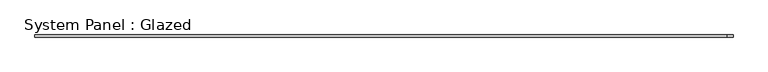
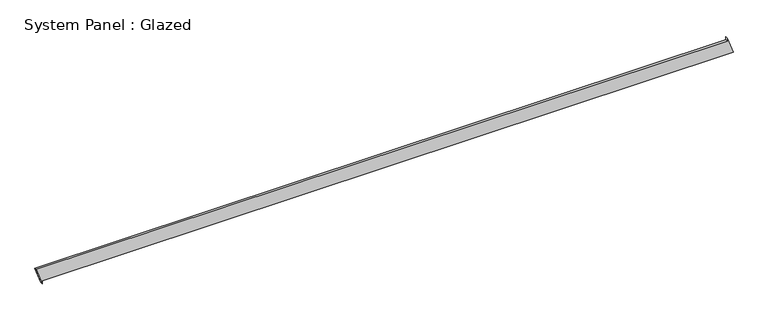
"""IFC4 building model written with IfcOpenShell, lengths in millimetres: plate geometry, System Panel : Glazed."""

from ifc_helpers import new_model, si_unit, frame, origin, place, context, project, spatial, polyline, outline, extrude, source, transform, mapped, element, save


def system_panel_glazed_df41a6c8(model_context):
    return source(origin(), model_context, "Body", "SweptSolid", [
        extrude(outline(polyline([(0.0, -3958.5507161), (35.3553391, -3958.5507161), (35.3553391, 4027.4801939), (234.7895843, 3958.8960097), (199.4342452, 3958.8966426), (199.2912695, -4027.4801939), (0.0, -3958.5507161)])), frame((0.0, -49.5, 0.0), z_axis=(0.0, 1.0, 0.0), x_axis=(0.0, 0.0, 1.0)), (0.0, 0.0, 1.0), 25.0),
    ])


if __name__ == "__main__":
    model = new_model("IFC4")
    model_context = context("Model", 3, world=origin())
    ifc_project = project(units=[si_unit("LENGTHUNIT", "METRE", prefix="MILLI")], contexts=[model_context])
    site = spatial("IfcSite", under=ifc_project)
    building = spatial("IfcBuilding", under=site)
    placement = place(None, origin())
    system_panel_glazed_shape = system_panel_glazed_df41a6c8(model_context)
    element("IfcPlate", 1, ObjectType="System Panel : Glazed", at=placement, inside=building, context=model_context, shape_type="MappedRepresentation", body=[
        mapped(system_panel_glazed_shape, transform((0.0, 0.0, 0.0), x_axis=(1.0, 0.0, 0.0), y_axis=(0.0, 1.0, 0.0), z_axis=(0.0, 0.0, 1.0))),
    ])
    save(model, "model.ifc")

# Revit data of these elements
# Element 1 (IfcPlate, "System Panel : Glazed")
#   Materials on its faces: "Glass"
# Materials
#   "Glass": class "Glass", colour RGB 218 227 224, transparency 0.85, Description = "Soda Lime Glass", Cost = 0
